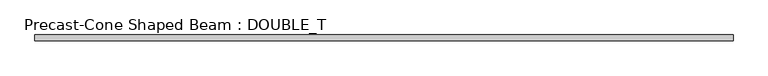
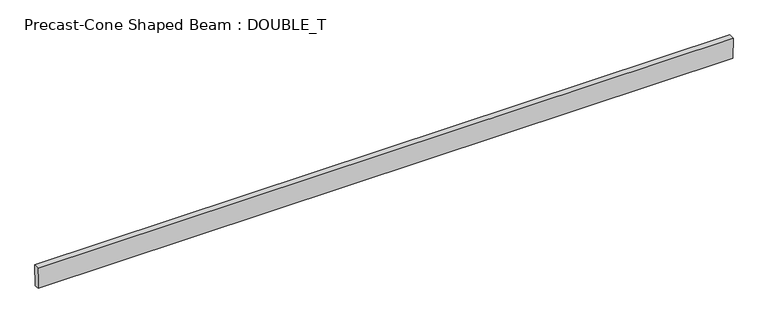
"""IFC4 building model written with IfcOpenShell, lengths in millimetres: beam geometry, Precast-Cone Shaped Beam : DOUBLE_T."""

from ifc_helpers import new_model, si_unit, frame, origin, place, context, project, spatial, polyline, outline, extrude, source, transform, mapped, element, save


def precast_cone_shaped_beam_double_t_64f85e83(model_context):
    return source(origin(), model_context, "Body", "SweptSolid", [
        extrude(outline(polyline([(-50.8, -228.6), (-63.5, 228.6), (63.5, 228.6), (50.8, -228.6), (-50.8, -228.6)])), frame((-7391.4, 0.0, 0.0), z_axis=(1.0, 0.0, 0.0), x_axis=(0.0, 1.0, 0.0)), (0.0, 0.0, 1.0), 14770.1),
    ])


if __name__ == "__main__":
    model = new_model("IFC4")
    model_context = context("Model", 3, world=origin())
    ifc_project = project(units=[si_unit("LENGTHUNIT", "METRE", prefix="MILLI")], contexts=[model_context])
    site = spatial("IfcSite", under=ifc_project)
    building = spatial("IfcBuilding", under=site)
    placement = place(None, origin())
    precast_cone_shaped_beam_double_t_shape = precast_cone_shaped_beam_double_t_64f85e83(model_context)
    element("IfcBeam", 1, ObjectType="Precast-Cone Shaped Beam : DOUBLE_T", at=placement, inside=building, context=model_context, shape_type="MappedRepresentation", body=[
        mapped(precast_cone_shaped_beam_double_t_shape, transform((0.0, 0.0, 0.0), x_axis=(1.0, 0.0, 0.0), y_axis=(0.0, 1.0, 0.0), z_axis=(0.0, 0.0, 1.0))),
    ])
    save(model, "model.ifc")

# Revit data of these elements
# Type "Precast-Cone Shaped Beam : DOUBLE_T"
#   Top Width = 0' - 5"
#   Tie Rod Weight [instance default] = 30
#   Tie Rod W [instance default] = 0.0660938 kip
#   Single Rebar Weight [instance default] = 50
#   Single Rebar W [instance default] = 0.110156 kip
#   Rebar Grids Weight [instance default] = 100
#   Rebar Grids W [instance default] = 0.220313 kip
#   Depth = 1' - 6"
#   Bottom Width = 0' - 4"
#   Length [instance default] = 5' - 0"
#   Structural Material [instance default] = Concrete, Precast
#   Assembly Code = ""
# Element 1 (IfcBeam, "Precast-Cone Shaped Beam : DOUBLE_T")
#   Length = 49' - 6"
#   Structural Material = Concrete - Precast Concrete - Normal Weight Concrete - 5 ksi
#   Materials on its faces: "Concrete - Precast Concrete - Normal Weight Concrete - 5 ksi"
# Materials
#   "Concrete, Precast": class "Concrete", colour RGB 198 187 187, transparency 0, Description = "Precast concrete", Cost = 0
#   "Concrete - Precast Concrete - Normal Weight Concrete - 5 ksi": class "Concrete", colour RGB 198 187 187, transparency 0, Cost = 0
